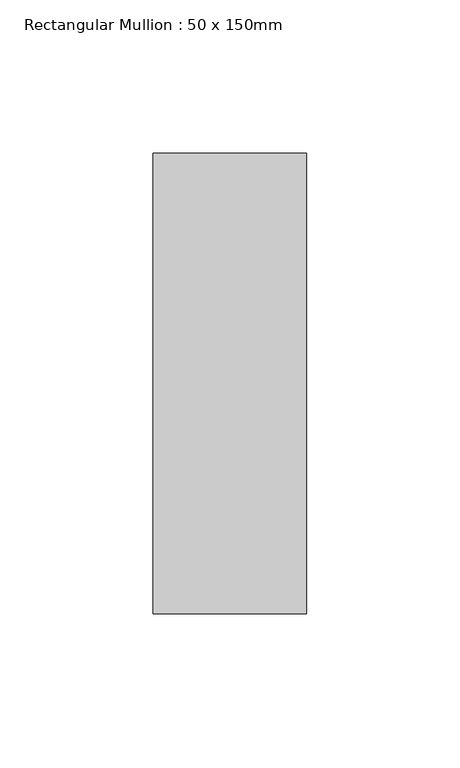
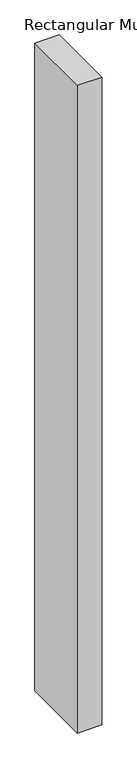
"""IFC4 building model written with IfcOpenShell, lengths in millimetres: member geometry, Rectangular Mullion : 50 x 150mm."""

import ifcopenshell
import ifcopenshell.guid

model = None  # the IFC model being written
_history = None  # IfcOwnerHistory: only IFC2X3 demands one
_inside = {}  # id of a spatial element -> (the spatial element, [elements in it])
_under = {}  # id of a project, library or spatial element -> (it, [spatial elements below it])
_declared = {}  # id of a project -> (the project, [libraries it declares])
_typed = {}  # id of a type object -> (the type object, [elements of that type])
_made_of = {}  # id of a material, layer set ... -> (it, [elements and type objects made of it])


def new_model(schema):
    """Start an empty IFC model of exactly this schema.

    Asked for "IFC4X3", IfcOpenShell would pick the latest addendum, in which some entities
    have other attributes; the version numbers below select the first issue.
    IFC2X3 requires an IfcOwnerHistory on every rooted entity: one is made here for all.
    """
    global model, _history
    if schema == "IFC4X3":
        model = ifcopenshell.file(schema_version=(4, 3, 0, 0))
    else:
        model = ifcopenshell.file(schema=schema)
    _inside.clear()
    _under.clear()
    _declared.clear()
    _typed.clear()
    _made_of.clear()
    _history = None
    if model.schema == "IFC2X3":
        org = make("IfcOrganization", Name="unknown")
        user = make(
            "IfcPersonAndOrganization",
            ThePerson=make("IfcPerson", FamilyName="unknown"),
            TheOrganization=org,
        )
        app = make(
            "IfcApplication",
            ApplicationDeveloper=org,
            Version="unknown",
            ApplicationFullName="unknown",
            ApplicationIdentifier="unknown",
        )
        _history = make(
            "IfcOwnerHistory",
            OwningUser=user,
            OwningApplication=app,
            ChangeAction="ADDED",
            CreationDate=0,
        )
    return model


def make(cls, **values):
    """One entity of the class cls with the attributes given. An attribute that is None is left unset."""
    return model.create_entity(
        cls, **{name: value for name, value in values.items() if value is not None}
    )


def rooted(cls, **values):
    """An entity with a GlobalId (a new one), such as an element, a storey or a relation."""
    return make(cls, GlobalId=ifcopenshell.guid.new(), OwnerHistory=_history, **values)


def si_unit(unit_type, name, prefix=None):
    """IfcSIUnit, for example si_unit("LENGTHUNIT", "METRE", prefix="MILLI")."""
    return make("IfcSIUnit", UnitType=unit_type, Prefix=prefix, Name=name)


def assignment(units):
    """IfcUnitAssignment: the units of a project."""
    return None if units is None else make("IfcUnitAssignment", Units=units)


def point(xyz):
    """IfcCartesianPoint."""
    return None if xyz is None else make("IfcCartesianPoint", Coordinates=xyz)


def direction(xyz):
    """IfcDirection."""
    return None if xyz is None else make("IfcDirection", DirectionRatios=xyz)


def frame(location, z_axis=None, x_axis=None):
    """IfcAxis2Placement3D, a coordinate frame: its origin and axes. An axis left out is left unset."""
    return make(
        "IfcAxis2Placement3D",
        Location=point(location),
        Axis=direction(z_axis),
        RefDirection=direction(x_axis),
    )


def origin():
    """The frame at (0, 0, 0) with its axes left unset."""
    return frame((0.0, 0.0, 0.0))


def place(relative_to, where):
    """IfcLocalPlacement: puts the frame where relative to a parent placement (None: the world)."""
    return make(
        "IfcLocalPlacement", PlacementRelTo=relative_to, RelativePlacement=where
    )


def context(
    kind, dimensions, precision=None, world=None, true_north=None, identifier=None
):
    """IfcGeometricRepresentationContext, for example the 3D "Model" context."""
    return make(
        "IfcGeometricRepresentationContext",
        ContextIdentifier=identifier,
        ContextType=kind,
        CoordinateSpaceDimension=dimensions,
        Precision=precision,
        WorldCoordinateSystem=world,
        TrueNorth=true_north,
    )


def project(units=None, contexts=None):
    """IfcProject with its units and contexts."""
    return rooted(
        "IfcProject",
        Name="project",
        RepresentationContexts=contexts,
        UnitsInContext=assignment(units),
    )


def spatial(cls, under=None, at=None, **own):
    """A site, building, storey or space (cls), placed at a placement, below another one or the project."""
    s = rooted(cls, ObjectPlacement=at, **own)
    if under is not None:
        _under.setdefault(under.id(), (under, []))[1].append(s)
    return s


def polyline(points):
    """IfcPolyline through the points."""
    return make("IfcPolyline", Points=[point(p) for p in points])


def outline(outer, holes=None, kind="AREA"):
    """IfcArbitraryClosedProfileDef: a profile drawn as a closed curve; with holes, ...WithVoids."""
    if holes is None:
        return make("IfcArbitraryClosedProfileDef", ProfileType=kind, OuterCurve=outer)
    return make(
        "IfcArbitraryProfileDefWithVoids",
        ProfileType=kind,
        OuterCurve=outer,
        InnerCurves=holes,
    )


def extrude(swept, where, along, depth):
    """IfcExtrudedAreaSolid: the profile swept, set in the frame where, extruded along a direction by depth."""
    return make(
        "IfcExtrudedAreaSolid",
        SweptArea=swept,
        Position=where,
        ExtrudedDirection=direction(along),
        Depth=depth,
    )


def shape(context_of_items, identifier, shape_type, items):
    """IfcShapeRepresentation: the items that make up one representation, for example the "Body"."""
    return make(
        "IfcShapeRepresentation",
        ContextOfItems=context_of_items,
        RepresentationIdentifier=identifier,
        RepresentationType=shape_type,
        Items=items,
    )


def source(mapping_origin, context_of_items, identifier, shape_type, items):
    """IfcRepresentationMap: a shape defined once, which mapped items show again and again."""
    return make(
        "IfcRepresentationMap",
        MappingOrigin=mapping_origin,
        MappedRepresentation=shape(context_of_items, identifier, shape_type, items),
    )


def transform(
    local_origin,
    x_axis=None,
    y_axis=None,
    z_axis=None,
    scale=None,
    scale2=None,
    scale3=None,
    uniform=True,
):
    """IfcCartesianTransformationOperator3D, or its non-uniform kind. x_axis, y_axis, z_axis: its Axis1, 2, 3."""
    if uniform:
        return make(
            "IfcCartesianTransformationOperator3D",
            Axis1=direction(x_axis),
            Axis2=direction(y_axis),
            LocalOrigin=point(local_origin),
            Scale=scale,
            Axis3=direction(z_axis),
        )
    return make(
        "IfcCartesianTransformationOperator3DnonUniform",
        Axis1=direction(x_axis),
        Axis2=direction(y_axis),
        LocalOrigin=point(local_origin),
        Scale=scale,
        Axis3=direction(z_axis),
        Scale2=scale2,
        Scale3=scale3,
    )


def mapped(mapping_source, mapping_target):
    """IfcMappedItem: shows the shape of a source again, moved by a transform."""
    return make(
        "IfcMappedItem", MappingSource=mapping_source, MappingTarget=mapping_target
    )


def made_of(thing, what):
    """Note that an element or type object is made of a material, layer set ...; save() writes the relation."""
    if what is not None:
        _made_of.setdefault(what.id(), (what, []))[1].append(thing)
    return thing


def element(
    cls,
    number,
    at=None,
    inside=None,
    cuts=None,
    type_object=None,
    material=None,
    context=None,
    identifier="Body",
    shape_type=None,
    held_by="IfcProductDefinitionShape",
    body=None,
    shapes=None,
    **own,
):
    """One element of the class cls, such as IfcWall. Its Tag is "e" and its number.

    at: its placement. inside: the storey or other place that contains it. cuts: it is an
    opening in that element (IfcRelVoidsElement). A single representation is given by context,
    identifier, shape_type and body (its items); several are given by shapes. held_by: the class
    of the entity that holds the representations. save() writes the other relations.
    """
    e = rooted(cls, Tag="e%d" % number, ObjectPlacement=at, **own)
    if body is not None:
        shapes = [shape(context, identifier, shape_type, body)]
    if shapes is not None:
        e.Representation = make(held_by, Representations=shapes)
    if inside is not None:
        _inside.setdefault(inside.id(), (inside, []))[1].append(e)
    if cuts is not None:
        rooted(
            "IfcRelVoidsElement", RelatingBuildingElement=cuts, RelatedOpeningElement=e
        )
    if type_object is not None:
        _typed.setdefault(type_object.id(), (type_object, []))[1].append(e)
    return made_of(e, material)


def aggregate(whole, parts):
    """IfcRelAggregates: a whole, such as a stair, and the parts it consists of."""
    return rooted("IfcRelAggregates", RelatingObject=whole, RelatedObjects=parts)


def save(model, path):
    """Write the relations noted so far, then the file.

    IfcRelAggregates (storeys below a building ...), IfcRelContainedInSpatialStructure (elements
    in a storey), IfcRelDefinesByType, IfcRelAssociatesMaterial and IfcRelDeclares: one each for
    every whole, place, type object, material and project.
    """
    for whole, parts in _under.values():
        aggregate(whole, parts)
    for where, things in _inside.values():
        rooted(
            "IfcRelContainedInSpatialStructure",
            RelatedElements=things,
            RelatingStructure=where,
        )
    for kind, things in _typed.values():
        rooted("IfcRelDefinesByType", RelatedObjects=things, RelatingType=kind)
    for what, things in _made_of.values():
        rooted("IfcRelAssociatesMaterial", RelatedObjects=things, RelatingMaterial=what)
    for by, libraries in _declared.values():
        rooted("IfcRelDeclares", RelatingContext=by, RelatedDefinitions=libraries)
    model.write(path)


def rectangular_mullion_50_x_150mm_0ac3c94c(model_context):
    return source(origin(), model_context, "Body", "SweptSolid", [
        extrude(outline(polyline([(0.0, 75.0), (0.0, -75.0), (-50.0, -75.0), (-50.0, 75.0), (0.0, 75.0)])), frame((0.0, 0.0, -1400.0), z_axis=(0.0, 0.0, 1.0), x_axis=(1.0, 0.0, 0.0)), (0.0, 0.0, 1.0), 1400.0),
    ])


if __name__ == "__main__":
    model = new_model("IFC4")
    model_context = context("Model", 3, world=origin())
    ifc_project = project(units=[si_unit("LENGTHUNIT", "METRE", prefix="MILLI")], contexts=[model_context])
    site = spatial("IfcSite", under=ifc_project)
    building = spatial("IfcBuilding", under=site)
    placement = place(None, origin())
    rectangular_mullion_50_x_150mm_shape = rectangular_mullion_50_x_150mm_0ac3c94c(model_context)
    element("IfcMember", 1, ObjectType="Rectangular Mullion : 50 x 150mm", at=placement, inside=building, context=model_context, shape_type="MappedRepresentation", body=[
        mapped(rectangular_mullion_50_x_150mm_shape, transform((0.0, 0.0, 0.0), x_axis=(1.0, 0.0, 0.0), y_axis=(0.0, 1.0, 0.0), z_axis=(0.0, 0.0, 1.0))),
    ])
    save(model, "model.ifc")

# Revit data of these elements
# Type "Rectangular Mullion : 50 x 150mm"
#   built-in parameter 1007304 = 0.492126 (stored number, unit not read)
#   built-in parameter 1007301 = 0.082021 (stored number, unit not read)
#   built-in parameter 1007300 = 0.082021 (stored number, unit not read)
# Element 1 (IfcMember, "Rectangular Mullion : 50 x 150mm")
#   Materials on its faces: "Metal - Aluminium"
# Materials
#   "Metal - Aluminium": class "Metal", colour RGB 247 247 247, transparency 0
